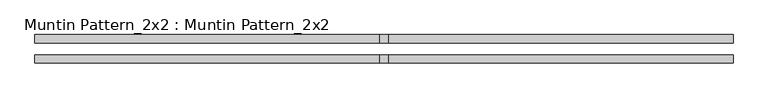
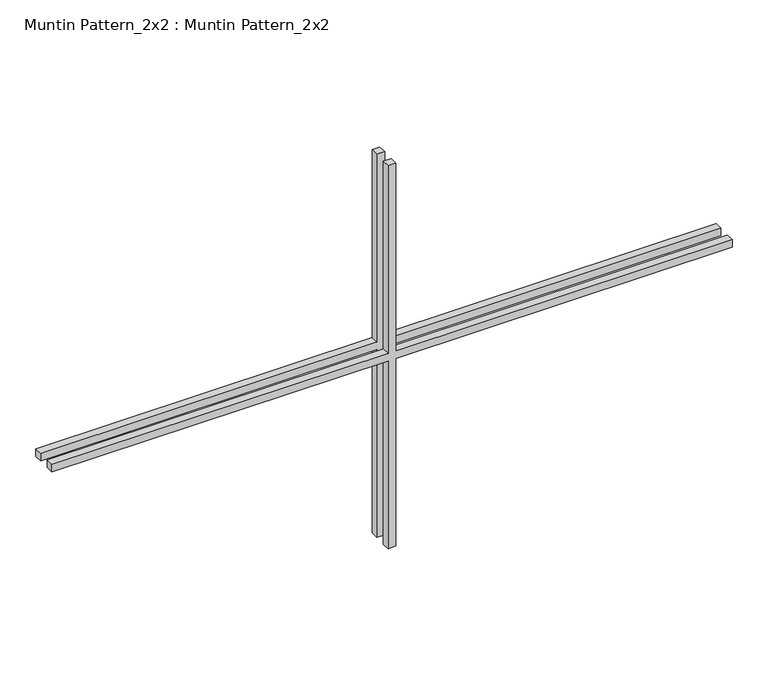
"""IFC4 building model written with IfcOpenShell, lengths in millimetres: proxy geometry, Muntin Pattern_2x2 : Muntin Pattern_2x2."""

from ifc_helpers import new_model, si_unit, frame, origin, place, context, project, spatial, polyline, outline, extrude, source, transform, mapped, element, save


def muntin_pattern_2x2_muntin_pattern_2x2_2b08dfa8(model_context):
    return source(origin(), model_context, "Body", "SweptSolid", [
        extrude(outline(polyline([(331.7875, -6.35), (331.7875, -546.1), (319.0875, -546.1), (319.0875, -6.35), (0.0, -6.35), (0.0, 6.35), (319.0875, 6.35), (319.0875, 546.1), (331.7875, 546.1), (331.7875, 6.35), (650.875, 6.35), (650.875, -6.35), (331.7875, -6.35)])), frame((0.0, 9.525, 0.0), z_axis=(0.0, 1.0, 0.0), x_axis=(0.0, 0.0, 1.0)), (0.0, 0.0, 1.0), 12.7),
        extrude(outline(polyline([(331.7875, -6.35), (331.7875, -546.1), (319.0875, -546.1), (319.0875, -6.35), (0.0, -6.35), (0.0, 6.35), (319.0875, 6.35), (319.0875, 546.1), (331.7875, 546.1), (331.7875, 6.35), (650.875, 6.35), (650.875, -6.35), (331.7875, -6.35)])), frame((0.0, -22.225, 0.0), z_axis=(0.0, 1.0, 0.0), x_axis=(0.0, 0.0, 1.0)), (0.0, 0.0, 1.0), 12.7),
    ])


if __name__ == "__main__":
    model = new_model("IFC4")
    model_context = context("Model", 3, world=origin())
    ifc_project = project(units=[si_unit("LENGTHUNIT", "METRE", prefix="MILLI")], contexts=[model_context])
    site = spatial("IfcSite", under=ifc_project)
    building = spatial("IfcBuilding", under=site)
    placement = place(None, origin())
    muntin_pattern_2x2_muntin_pattern_2x2_shape = muntin_pattern_2x2_muntin_pattern_2x2_2b08dfa8(model_context)
    element("IfcBuildingElementProxy", 1, Name="Muntin Pattern_2x2 : Muntin Pattern_2x2", ObjectType="Muntin Pattern_2x2 : Muntin Pattern_2x2", at=placement, inside=building, context=model_context, shape_type="MappedRepresentation", body=[
        mapped(muntin_pattern_2x2_muntin_pattern_2x2_shape, transform((0.0, 0.0, 0.0), x_axis=(1.0, 0.0, 0.0), y_axis=(0.0, 1.0, 0.0), z_axis=(0.0, 0.0, 1.0))),
    ])
    save(model, "model.ifc")

# Revit data of these elements
# Type "Muntin Pattern_2x2 : Muntin Pattern_2x2"
#   Width [instance default] = 4' - 0"
#   Thickness = 0' - 0 1/2"
#   Height [instance default] = 4' - 0"
#   Distance = 0' - 0 3/4"
#   Interior Material [instance default] = none
#   Exterior Material [instance default] = none
# Element 1 (IfcBuildingElementProxy, "Muntin Pattern_2x2 : Muntin Pattern_2x2")
#   Width = 3' - 7"
#   Height = 2' - 1 5/8"
#   Interior Material = Wood - Stained
#   Exterior Material = Clad - White
#   Materials on its faces: "Clad - White", "Wood - Stained"
# Materials
#   "Clad - White": class "Wood", colour RGB 242 242 238, transparency 0, Cost = 0
#   "Wood - Stained": class "Wood", colour RGB 224 178 126, transparency 0, Cost = 0
